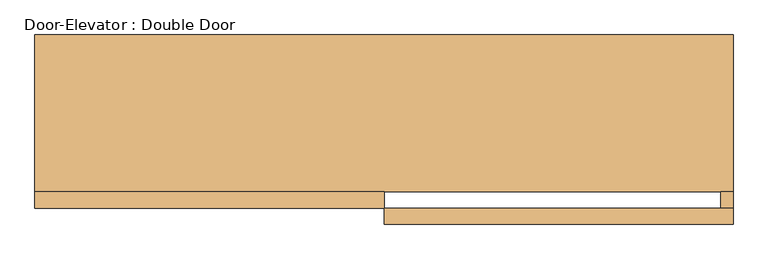
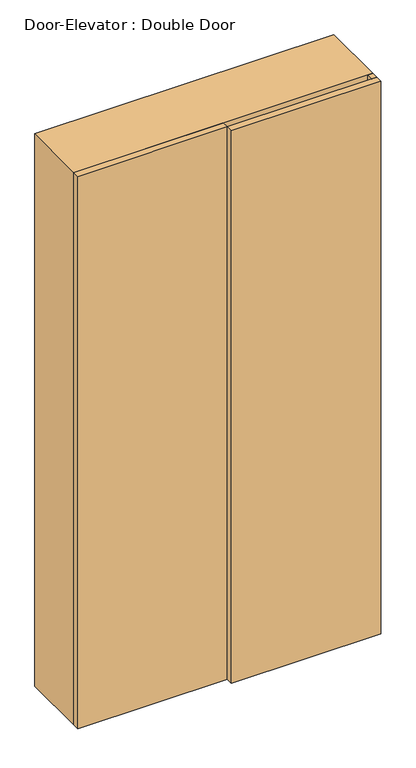
"""IFC4 building model written with IfcOpenShell, lengths in millimetres: door geometry, Door-Elevator : Double Door."""

from ifc_helpers import new_model, si_unit, frame, origin, origin_with_axes, place, context, project, spatial, polyline, outline, extrude, source, transform, mapped, element, save


def door_elevator_double_door_0d043116(model_context):
    return source(origin(), model_context, "Body", "SweptSolid", [
        extrude(outline(polyline([(546.1, -182.15), (546.1, -207.55), (0.0, -207.55), (0.0, -182.15), (546.1, -182.15)])), origin_with_axes(), (0.0, 0.0, 1.0), 2133.6),
        extrude(outline(polyline([(0.0, -156.75), (0.0, -182.15), (-546.1, -182.15), (-546.1, -156.75), (0.0, -156.75)])), origin_with_axes(), (0.0, 0.0, 1.0), 2133.6),
        extrude(outline(polyline([(546.1, -156.75), (546.1, -182.15), (527.05, -182.15), (527.05, -156.75), (546.1, -156.75)])), origin_with_axes(), (0.0, 0.0, 1.0), 2133.6),
        extrude(outline(polyline([(0.0, -527.05), (2114.55, -527.05), (2114.55, 527.05), (0.0, 527.05), (0.0, 546.1), (2133.6, 546.1), (2133.6, -546.1), (0.0, -546.1), (0.0, -527.05)])), frame((0.0, -156.75, 0.0), z_axis=(0.0, 1.0, 0.0), x_axis=(0.0, 0.0, 1.0)), (0.0, 0.0, 1.0), 245.65),
    ])


if __name__ == "__main__":
    model = new_model("IFC4")
    model_context = context("Model", 3, world=origin())
    ifc_project = project(units=[si_unit("LENGTHUNIT", "METRE", prefix="MILLI")], contexts=[model_context])
    site = spatial("IfcSite", under=ifc_project)
    building = spatial("IfcBuilding", under=site)
    placement = place(None, origin())
    door_elevator_double_door_shape = door_elevator_double_door_0d043116(model_context)
    element("IfcDoor", 1, ObjectType="Door-Elevator : Double Door", at=placement, inside=building, context=model_context, shape_type="MappedRepresentation", body=[
        mapped(door_elevator_double_door_shape, transform((0.0, 0.0, 0.0), x_axis=(1.0, 0.0, 0.0), y_axis=(0.0, 1.0, 0.0), z_axis=(0.0, 0.0, 1.0))),
    ])
    save(model, "model.ifc")

# Revit data of these elements
# Type "Door-Elevator : Double Door"
#   Type Mark = "EX5-"
#   P_WWSKU = ""
#   Filter Visibiilty = "Existing Elevator"
#   Analytic Construction = "<None>"
#   Trim Projection = 12.7 mm
#   Thickness = 25.4 mm
#   Height = 2133.6 mm
#   Trim Width = 19.05 mm
#   Width = 1092.2 mm
#   Door_Quad = 273.05 mm
#   Door_Double = 546.1 mm
#   Cab Width = 1828.8 mm
#   Cab Offset [instance default] = 0 mm
#   Cab Depth = 1828.8 mm
#   _factor4 = 4
#   _factor2 = 2
#   WW-HardwareSet [instance default] = 0
#   Simple Plan = yes
#   Quad = no
#   Plan Lines [instance default] = yes
#   Double = yes
#   Panel Type = element 9002524
#   Type Comments = ""
#   Keynote = ""
#   Function = (empty or 0)
#   Wall Closure = (empty or 0)
#   Assembly Code = ""
# Element 1 (IfcDoor, "Door-Elevator : Double Door")
#   Materials on its faces: "WW-EC-RGB-White"
# Materials
#   "WW-EC-RGB-White": class "Generic", colour RGB 255 255 255, transparency 0, Comments = "If region requests off-white, swith asset color to RGB 231-228-220", Description = "Generic Color", Cost = 0
